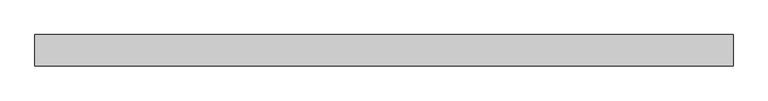
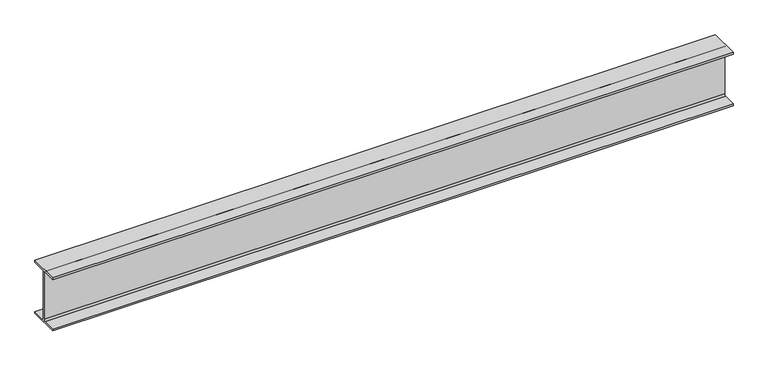
"""IFC4 building model written with IfcOpenShell, lengths in millimetres: beam geometry, Steel Beam_H-KSD3502 : H_SB_ASB_H-200x200x8x12."""

from ifc_helpers import new_model, si_unit, point, frame, frame_2d, origin, place, context, project, spatial, polyline, circle_curve, trimmed, segment, composite_curve, outline, extrude, source, transform, mapped, element, save


def beam_556eb451(model_context):
    return source(origin(), model_context, "Body", "SweptSolid", [
        extrude(outline(composite_curve([segment(polyline([(-82.5, -141.5), (-11.9, -141.5)]), True, "CONTINUOUS"), segment(trimmed(circle_curve(frame_2d((-11.9, -132.6)), 8.9), [point((-11.9, -141.5))], [point((-3.0, -132.6))], True, "CARTESIAN"), True, "CONTINUOUS"), segment(polyline([(-3.0, -132.6), (-3.0, 132.6)]), True, "CONTINUOUS"), segment(trimmed(circle_curve(frame_2d((-11.9, 132.6)), 8.9), [point((-3.0, 132.6))], [point((-11.9, 141.5))], True, "CARTESIAN"), True, "CONTINUOUS"), segment(polyline([(-11.9, 141.5), (-82.5, 141.5), (-82.5, 151.7), (82.5, 151.7), (82.5, 141.5), (11.9, 141.5)]), True, "CONTINUOUS"), segment(trimmed(circle_curve(frame_2d((11.9, 132.6)), 8.9), [point((11.9, 141.5))], [point((3.0, 132.6))], True, "CARTESIAN"), True, "CONTINUOUS"), segment(polyline([(3.0, 132.6), (3.0, -132.6)]), True, "CONTINUOUS"), segment(trimmed(circle_curve(frame_2d((11.9, -132.6)), 8.9), [point((3.0, -132.6))], [point((11.9, -141.5))], True, "CARTESIAN"), True, "CONTINUOUS"), segment(polyline([(11.9, -141.5), (82.5, -141.5), (82.5, -151.7), (-82.5, -151.7), (-82.5, -141.5)]), True, "CONTINUOUS")], self_intersect=False)), frame((-1848.779151, 0.0, 0.0), z_axis=(1.0, 0.0, 0.0), x_axis=(0.0, 1.0, 0.0)), (0.0, 0.0, 1.0), 3672.4688696),
    ])


if __name__ == "__main__":
    model = new_model("IFC4")
    model_context = context("Model", 3, world=origin())
    ifc_project = project(units=[si_unit("LENGTHUNIT", "METRE", prefix="MILLI")], contexts=[model_context])
    site = spatial("IfcSite", under=ifc_project)
    building = spatial("IfcBuilding", under=site)
    placement = place(None, origin())
    beam_shape = beam_556eb451(model_context)
    element("IfcBeam", 1, ObjectType="Steel Beam_H-KSD3502 : H_SB_ASB_H-200x200x8x12", at=placement, inside=building, context=model_context, shape_type="MappedRepresentation", body=[
        mapped(beam_shape, transform((0.0, 0.0, 0.0), x_axis=(1.0, 0.0, 0.0), y_axis=(0.0, 1.0, 0.0), z_axis=(0.0, 0.0, 1.0))),
    ])
    save(model, "model.ifc")

# Revit data of these elements
# Type "Steel Beam_H-KSD3502 : H_SB_ASB_H-200x200x8x12"
#   Width = 20.0 cm
#   Web Thickness = 0.8 cm
#   Web Fillet = 1.3 cm
#   Warping Constant = 141376.0 cm⁶
#   Torsional Moment of Inertia = 26.2485 cm⁴
#   Torsional Modulus = 1.0 cm³
#   Section Area = 63.53 cm²
#   Plastic Modulus weak axis = 244.0 cm³
#   Plastic Modulus strong axis = 525.0 cm³
#   Perimeter = 1.16 m²/m
#   Nominal Weight = 49.90 kgf/m
#   Moment of Inertia weak axis = 1600.00 cm⁴
#   Moment of Inertia strong axis = 4720.00 cm⁴
#   Height = 20.0 cm
#   Flange Thickness = 1.2 cm
#   Elastic Modulus weak axis = 160.0 cm³
#   Elastic Modulus strong axis = 472.0 cm³
#   Centroid Vertical = 10.0 cm
#   Centroid Horizontal = 10.0 cm
#   Length [instance default] = 1.5240 m
#   Structural Material [instance default] = Steel, 45-345
#   Assembly Code = ""
# Element 1 (IfcBeam, "Steel Beam_H-KSD3502 : H_SB_ASB_H-200x200x8x12")
#   Structural Material = none
# Materials
#   "Steel, 45-345": class "Metal", colour RGB 189 187 185, transparency 0, Description = "Steel 345 MPa", Cost = 0
